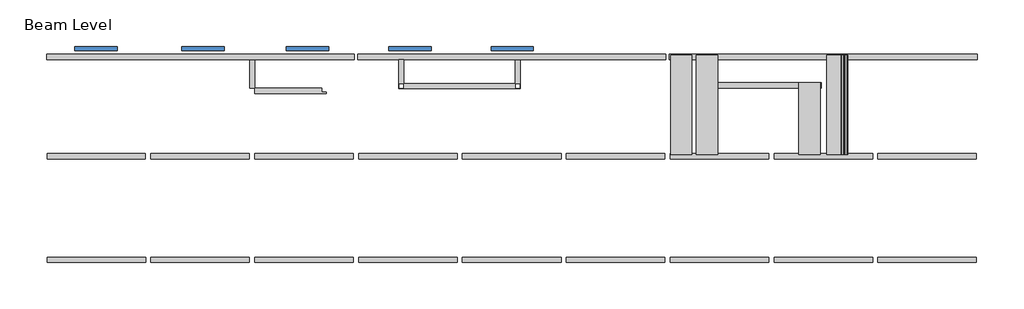
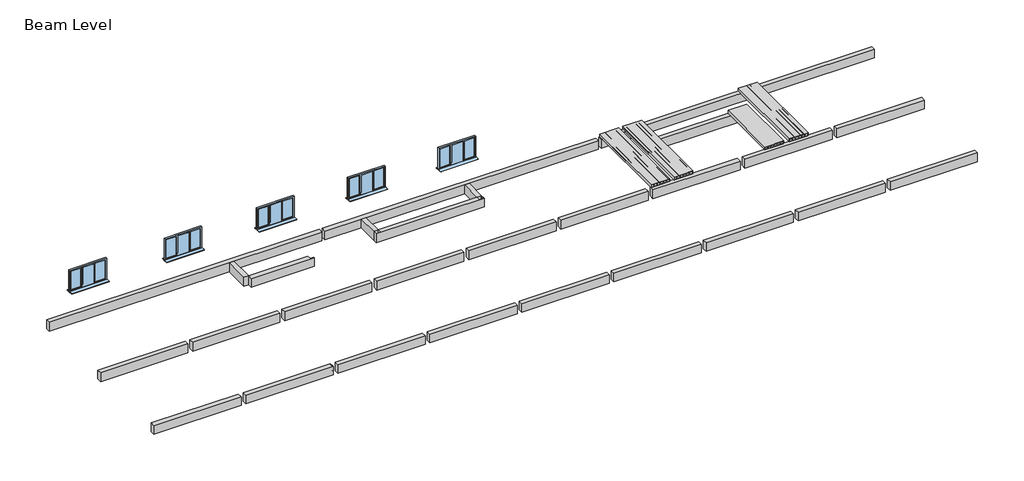
# One storey: 28 beams, 5 windows, 4 proxies.
"""IFC4 building model written with IfcOpenShell, lengths in millimetres."""

import ifcopenshell
import ifcopenshell.guid

model = None  # the IFC model being written
_history = None  # IfcOwnerHistory: only IFC2X3 demands one
_inside = {}  # id of a spatial element -> (the spatial element, [elements in it])
_under = {}  # id of a project, library or spatial element -> (it, [spatial elements below it])
_declared = {}  # id of a project -> (the project, [libraries it declares])
_typed = {}  # id of a type object -> (the type object, [elements of that type])
_made_of = {}  # id of a material, layer set ... -> (it, [elements and type objects made of it])


def new_model(schema):
    """Start an empty IFC model of exactly this schema.

    Asked for "IFC4X3", IfcOpenShell would pick the latest addendum, in which some entities
    have other attributes; the version numbers below select the first issue.
    IFC2X3 requires an IfcOwnerHistory on every rooted entity: one is made here for all.
    """
    global model, _history
    if schema == "IFC4X3":
        model = ifcopenshell.file(schema_version=(4, 3, 0, 0))
    else:
        model = ifcopenshell.file(schema=schema)
    _inside.clear()
    _under.clear()
    _declared.clear()
    _typed.clear()
    _made_of.clear()
    _history = None
    if model.schema == "IFC2X3":
        org = make("IfcOrganization", Name="unknown")
        user = make(
            "IfcPersonAndOrganization",
            ThePerson=make("IfcPerson", FamilyName="unknown"),
            TheOrganization=org,
        )
        app = make(
            "IfcApplication",
            ApplicationDeveloper=org,
            Version="unknown",
            ApplicationFullName="unknown",
            ApplicationIdentifier="unknown",
        )
        _history = make(
            "IfcOwnerHistory",
            OwningUser=user,
            OwningApplication=app,
            ChangeAction="ADDED",
            CreationDate=0,
        )
    return model


def make(cls, **values):
    """One entity of the class cls with the attributes given. An attribute that is None is left unset."""
    return model.create_entity(
        cls, **{name: value for name, value in values.items() if value is not None}
    )


def rooted(cls, **values):
    """An entity with a GlobalId (a new one), such as an element, a storey or a relation."""
    return make(cls, GlobalId=ifcopenshell.guid.new(), OwnerHistory=_history, **values)


def si_unit(unit_type, name, prefix=None):
    """IfcSIUnit, for example si_unit("LENGTHUNIT", "METRE", prefix="MILLI")."""
    return make("IfcSIUnit", UnitType=unit_type, Prefix=prefix, Name=name)


def assignment(units):
    """IfcUnitAssignment: the units of a project."""
    return None if units is None else make("IfcUnitAssignment", Units=units)


def point(xyz):
    """IfcCartesianPoint."""
    return None if xyz is None else make("IfcCartesianPoint", Coordinates=xyz)


def direction(xyz):
    """IfcDirection."""
    return None if xyz is None else make("IfcDirection", DirectionRatios=xyz)


def frame(location, z_axis=None, x_axis=None):
    """IfcAxis2Placement3D, a coordinate frame: its origin and axes. An axis left out is left unset."""
    return make(
        "IfcAxis2Placement3D",
        Location=point(location),
        Axis=direction(z_axis),
        RefDirection=direction(x_axis),
    )


def frame_2d(location, x_axis=None):
    """IfcAxis2Placement2D, a coordinate frame in the plane: its origin and x axis."""
    return make(
        "IfcAxis2Placement2D", Location=point(location), RefDirection=direction(x_axis)
    )


def origin():
    """The frame at (0, 0, 0) with its axes left unset."""
    return frame((0.0, 0.0, 0.0))


def place(relative_to, where):
    """IfcLocalPlacement: puts the frame where relative to a parent placement (None: the world)."""
    return make(
        "IfcLocalPlacement", PlacementRelTo=relative_to, RelativePlacement=where
    )


def context(
    kind, dimensions, precision=None, world=None, true_north=None, identifier=None
):
    """IfcGeometricRepresentationContext, for example the 3D "Model" context."""
    return make(
        "IfcGeometricRepresentationContext",
        ContextIdentifier=identifier,
        ContextType=kind,
        CoordinateSpaceDimension=dimensions,
        Precision=precision,
        WorldCoordinateSystem=world,
        TrueNorth=true_north,
    )


def project(units=None, contexts=None):
    """IfcProject with its units and contexts."""
    return rooted(
        "IfcProject",
        Name="project",
        RepresentationContexts=contexts,
        UnitsInContext=assignment(units),
    )


def spatial(cls, under=None, at=None, **own):
    """A site, building, storey or space (cls), placed at a placement, below another one or the project."""
    s = rooted(cls, ObjectPlacement=at, **own)
    if under is not None:
        _under.setdefault(under.id(), (under, []))[1].append(s)
    return s


def polyline(points):
    """IfcPolyline through the points."""
    return make("IfcPolyline", Points=[point(p) for p in points])


def circle_curve(where, radius):
    """IfcCircle in the frame where."""
    return make("IfcCircle", Position=where, Radius=radius)


def trimmed(basis, trim1, trim2, sense, master):
    """IfcTrimmedCurve: the piece of a basis curve between two trims."""
    return make(
        "IfcTrimmedCurve",
        BasisCurve=basis,
        Trim1=trim1,
        Trim2=trim2,
        SenseAgreement=sense,
        MasterRepresentation=master,
    )


def segment(curve, same_sense, transition):
    """IfcCompositeCurveSegment."""
    return make(
        "IfcCompositeCurveSegment",
        Transition=transition,
        SameSense=same_sense,
        ParentCurve=curve,
    )


def composite_curve(segments, self_intersect=None):
    """IfcCompositeCurve: segments joined end to end."""
    return make("IfcCompositeCurve", Segments=segments, SelfIntersect=self_intersect)


def outline(outer, holes=None, kind="AREA"):
    """IfcArbitraryClosedProfileDef: a profile drawn as a closed curve; with holes, ...WithVoids."""
    if holes is None:
        return make("IfcArbitraryClosedProfileDef", ProfileType=kind, OuterCurve=outer)
    return make(
        "IfcArbitraryProfileDefWithVoids",
        ProfileType=kind,
        OuterCurve=outer,
        InnerCurves=holes,
    )


def extrude(swept, where, along, depth):
    """IfcExtrudedAreaSolid: the profile swept, set in the frame where, extruded along a direction by depth."""
    return make(
        "IfcExtrudedAreaSolid",
        SweptArea=swept,
        Position=where,
        ExtrudedDirection=direction(along),
        Depth=depth,
    )


def faces_of(points, faces, orient=None, outer=None):
    """IfcFace entities. A face is a list of loops; a loop is a list of indices into points, from 0.

    orient and outer hold one flag for each loop. By default every Orientation is true, the
    first loop of a face is its IfcFaceOuterBound and the others are IfcFaceBound.
    """
    made = []
    for i, loops in enumerate(faces):
        bounds = []
        for j, loop in enumerate(loops):
            is_outer = j == 0 if outer is None else outer[i][j]
            bounds.append(
                make(
                    "IfcFaceOuterBound" if is_outer else "IfcFaceBound",
                    Bound=make("IfcPolyLoop", Polygon=[points[k] for k in loop]),
                    Orientation=True if orient is None else orient[i][j],
                )
            )
        made.append(make("IfcFace", Bounds=bounds))
    return made


def faceted_brep(points, faces, orient=None, outer=None, voids=None):
    """IfcFacetedBrep: a solid bounded by flat faces; with voids (closed shells), ...WithVoids."""
    shared = [point(p) for p in points]
    hull = make("IfcClosedShell", CfsFaces=faces_of(shared, faces, orient, outer))
    if voids is None:
        return make("IfcFacetedBrep", Outer=hull)
    return make(
        "IfcFacetedBrepWithVoids",
        Outer=hull,
        Voids=[
            make(cls, CfsFaces=faces_of(shared, fs, o, b)) for cls, fs, o, b in voids
        ],
    )


def shape(context_of_items, identifier, shape_type, items):
    """IfcShapeRepresentation: the items that make up one representation, for example the "Body"."""
    return make(
        "IfcShapeRepresentation",
        ContextOfItems=context_of_items,
        RepresentationIdentifier=identifier,
        RepresentationType=shape_type,
        Items=items,
    )


def source(mapping_origin, context_of_items, identifier, shape_type, items):
    """IfcRepresentationMap: a shape defined once, which mapped items show again and again."""
    return make(
        "IfcRepresentationMap",
        MappingOrigin=mapping_origin,
        MappedRepresentation=shape(context_of_items, identifier, shape_type, items),
    )


def transform(
    local_origin,
    x_axis=None,
    y_axis=None,
    z_axis=None,
    scale=None,
    scale2=None,
    scale3=None,
    uniform=True,
):
    """IfcCartesianTransformationOperator3D, or its non-uniform kind. x_axis, y_axis, z_axis: its Axis1, 2, 3."""
    if uniform:
        return make(
            "IfcCartesianTransformationOperator3D",
            Axis1=direction(x_axis),
            Axis2=direction(y_axis),
            LocalOrigin=point(local_origin),
            Scale=scale,
            Axis3=direction(z_axis),
        )
    return make(
        "IfcCartesianTransformationOperator3DnonUniform",
        Axis1=direction(x_axis),
        Axis2=direction(y_axis),
        LocalOrigin=point(local_origin),
        Scale=scale,
        Axis3=direction(z_axis),
        Scale2=scale2,
        Scale3=scale3,
    )


def mapped(mapping_source, mapping_target):
    """IfcMappedItem: shows the shape of a source again, moved by a transform."""
    return make(
        "IfcMappedItem", MappingSource=mapping_source, MappingTarget=mapping_target
    )


def made_of(thing, what):
    """Note that an element or type object is made of a material, layer set ...; save() writes the relation."""
    if what is not None:
        _made_of.setdefault(what.id(), (what, []))[1].append(thing)
    return thing


def element(
    cls,
    number,
    at=None,
    inside=None,
    cuts=None,
    type_object=None,
    material=None,
    context=None,
    identifier="Body",
    shape_type=None,
    held_by="IfcProductDefinitionShape",
    body=None,
    shapes=None,
    **own,
):
    """One element of the class cls, such as IfcWall. Its Tag is "e" and its number.

    at: its placement. inside: the storey or other place that contains it. cuts: it is an
    opening in that element (IfcRelVoidsElement). A single representation is given by context,
    identifier, shape_type and body (its items); several are given by shapes. held_by: the class
    of the entity that holds the representations. save() writes the other relations.
    """
    e = rooted(cls, Tag="e%d" % number, ObjectPlacement=at, **own)
    if body is not None:
        shapes = [shape(context, identifier, shape_type, body)]
    if shapes is not None:
        e.Representation = make(held_by, Representations=shapes)
    if inside is not None:
        _inside.setdefault(inside.id(), (inside, []))[1].append(e)
    if cuts is not None:
        rooted(
            "IfcRelVoidsElement", RelatingBuildingElement=cuts, RelatedOpeningElement=e
        )
    if type_object is not None:
        _typed.setdefault(type_object.id(), (type_object, []))[1].append(e)
    return made_of(e, material)


def aggregate(whole, parts):
    """IfcRelAggregates: a whole, such as a stair, and the parts it consists of."""
    return rooted("IfcRelAggregates", RelatingObject=whole, RelatedObjects=parts)


def save(model, path):
    """Write the relations noted so far, then the file.

    IfcRelAggregates (storeys below a building ...), IfcRelContainedInSpatialStructure (elements
    in a storey), IfcRelDefinesByType, IfcRelAssociatesMaterial and IfcRelDeclares: one each for
    every whole, place, type object, material and project.
    """
    for whole, parts in _under.values():
        aggregate(whole, parts)
    for where, things in _inside.values():
        rooted(
            "IfcRelContainedInSpatialStructure",
            RelatedElements=things,
            RelatingStructure=where,
        )
    for kind, things in _typed.values():
        rooted("IfcRelDefinesByType", RelatedObjects=things, RelatingType=kind)
    for what, things in _made_of.values():
        rooted("IfcRelAssociatesMaterial", RelatedObjects=things, RelatingMaterial=what)
    for by, libraries in _declared.values():
        rooted("IfcRelDeclares", RelatingContext=by, RelatedDefinitions=libraries)
    model.write(path)


def asb_beams_300asb153_cd404b0f(model_context):
    return source(origin(), model_context, "Body", "SweptSolid", [
        extrude(outline(composite_curve([segment(polyline([(95.0, 174.0), (95.0, 150.0), (40.5, 150.0)]), True, "CONTINUOUS"), segment(trimmed(circle_curve(frame_2d((40.5, 123.0)), 27.0), [point((40.5, 150.0))], [point((13.5, 123.0))], True, "CARTESIAN"), True, "CONTINUOUS"), segment(polyline([(13.5, 123.0), (13.5, -85.0)]), True, "CONTINUOUS"), segment(trimmed(circle_curve(frame_2d((40.5, -85.0)), 27.0), [point((13.5, -85.0))], [point((40.5, -112.0))], True, "CARTESIAN"), True, "CONTINUOUS"), segment(polyline([(40.5, -112.0), (150.0, -112.0), (150.0, -136.0), (-150.0, -136.0), (-150.0, -112.0), (-40.5, -112.0)]), True, "CONTINUOUS"), segment(trimmed(circle_curve(frame_2d((-40.5, -85.0)), 27.0), [point((-40.5, -112.0))], [point((-13.5, -85.0))], True, "CARTESIAN"), True, "CONTINUOUS"), segment(polyline([(-13.5, -85.0), (-13.5, 123.0)]), True, "CONTINUOUS"), segment(trimmed(circle_curve(frame_2d((-40.5, 123.0)), 27.0), [point((-13.5, 123.0))], [point((-40.5, 150.0))], True, "CARTESIAN"), True, "CONTINUOUS"), segment(polyline([(-40.5, 150.0), (-95.0, 150.0), (-95.0, 174.0), (95.0, 174.0)]), True, "CONTINUOUS")], self_intersect=False)), frame((-176.5, 0.0, 0.0), z_axis=(1.0, 0.0, 0.0), x_axis=(0.0, 1.0, 0.0)), (0.0, 0.0, 1.0), 36.0),
    ])


def hollow_core_b1c9e8cf(model_context):
    return source(origin(), model_context, "Body", "SweptSolid", [
        extrude(outline(polyline([(-609.6, 100.0), (609.6, 100.0), (609.6, -100.0), (-609.6, -100.0), (-609.6, 100.0)]), holes=[composite_curve([segment(trimmed(circle_curve(frame_2d((508.0, 0.0)), 60.0), [point((448.0, 0.0))], [point((568.0, 0.0))], True, "CARTESIAN"), True, "CONTINUOUS"), segment(trimmed(circle_curve(frame_2d((508.0, 0.0)), 60.0), [point((568.0, 0.0))], [point((448.0, 0.0))], True, "CARTESIAN"), True, "CONTINUOUS")], self_intersect=False), composite_curve([segment(trimmed(circle_curve(frame_2d((-508.0, 0.0)), 60.0), [point((-568.0, 0.0))], [point((-448.0, 0.0))], True, "CARTESIAN"), True, "CONTINUOUS"), segment(trimmed(circle_curve(frame_2d((-508.0, 0.0)), 60.0), [point((-448.0, 0.0))], [point((-568.0, 0.0))], True, "CARTESIAN"), True, "CONTINUOUS")], self_intersect=False), composite_curve([segment(trimmed(circle_curve(frame_2d((304.8, 0.0)), 60.0), [point((244.8, 0.0))], [point((364.8, 0.0))], True, "CARTESIAN"), True, "CONTINUOUS"), segment(trimmed(circle_curve(frame_2d((304.8, 0.0)), 60.0), [point((364.8, 0.0))], [point((244.8, 0.0))], True, "CARTESIAN"), True, "CONTINUOUS")], self_intersect=False), composite_curve([segment(trimmed(circle_curve(frame_2d((101.6, 0.0)), 60.0), [point((41.6, 0.0))], [point((161.6, 0.0))], True, "CARTESIAN"), True, "CONTINUOUS"), segment(trimmed(circle_curve(frame_2d((101.6, 0.0)), 60.0), [point((161.6, 0.0))], [point((41.6, 0.0))], True, "CARTESIAN"), True, "CONTINUOUS")], self_intersect=False), composite_curve([segment(trimmed(circle_curve(frame_2d((-101.6, 0.0)), 60.0), [point((-161.6, 0.0))], [point((-41.6, 0.0))], True, "CARTESIAN"), True, "CONTINUOUS"), segment(trimmed(circle_curve(frame_2d((-101.6, 0.0)), 60.0), [point((-41.6, 0.0))], [point((-161.6, 0.0))], True, "CARTESIAN"), True, "CONTINUOUS")], self_intersect=False), composite_curve([segment(trimmed(circle_curve(frame_2d((-304.8, 0.0)), 60.0), [point((-364.8, 0.0))], [point((-244.8, 0.0))], True, "CARTESIAN"), True, "CONTINUOUS"), segment(trimmed(circle_curve(frame_2d((-304.8, 0.0)), 60.0), [point((-244.8, 0.0))], [point((-364.8, 0.0))], True, "CARTESIAN"), True, "CONTINUOUS")], self_intersect=False)]), frame((0.0, 0.0, 0.0), z_axis=(1.0, 0.0, 0.0), x_axis=(0.0, 1.0, 0.0)), (0.0, 0.0, 1.0), 5760.0),
    ])


def hollow_core_a6975cb3(model_context):
    return source(origin(), model_context, "Body", "SweptSolid", [
        extrude(outline(polyline([(-609.6, 100.0), (609.6, 100.0), (609.6, -100.0), (-609.6, -100.0), (-609.6, 100.0)]), holes=[composite_curve([segment(trimmed(circle_curve(frame_2d((508.0, 0.0)), 60.0), [point((448.0, 0.0))], [point((568.0, 0.0))], True, "CARTESIAN"), True, "CONTINUOUS"), segment(trimmed(circle_curve(frame_2d((508.0, 0.0)), 60.0), [point((568.0, 0.0))], [point((448.0, 0.0))], True, "CARTESIAN"), True, "CONTINUOUS")], self_intersect=False), composite_curve([segment(trimmed(circle_curve(frame_2d((-508.0, 0.0)), 60.0), [point((-568.0, 0.0))], [point((-448.0, 0.0))], True, "CARTESIAN"), True, "CONTINUOUS"), segment(trimmed(circle_curve(frame_2d((-508.0, 0.0)), 60.0), [point((-448.0, 0.0))], [point((-568.0, 0.0))], True, "CARTESIAN"), True, "CONTINUOUS")], self_intersect=False), composite_curve([segment(trimmed(circle_curve(frame_2d((304.8, 0.0)), 60.0), [point((244.8, 0.0))], [point((364.8, 0.0))], True, "CARTESIAN"), True, "CONTINUOUS"), segment(trimmed(circle_curve(frame_2d((304.8, 0.0)), 60.0), [point((364.8, 0.0))], [point((244.8, 0.0))], True, "CARTESIAN"), True, "CONTINUOUS")], self_intersect=False), composite_curve([segment(trimmed(circle_curve(frame_2d((101.6, 0.0)), 60.0), [point((41.6, 0.0))], [point((161.6, 0.0))], True, "CARTESIAN"), True, "CONTINUOUS"), segment(trimmed(circle_curve(frame_2d((101.6, 0.0)), 60.0), [point((161.6, 0.0))], [point((41.6, 0.0))], True, "CARTESIAN"), True, "CONTINUOUS")], self_intersect=False), composite_curve([segment(trimmed(circle_curve(frame_2d((-101.6, 0.0)), 60.0), [point((-161.6, 0.0))], [point((-41.6, 0.0))], True, "CARTESIAN"), True, "CONTINUOUS"), segment(trimmed(circle_curve(frame_2d((-101.6, 0.0)), 60.0), [point((-41.6, 0.0))], [point((-161.6, 0.0))], True, "CARTESIAN"), True, "CONTINUOUS")], self_intersect=False), composite_curve([segment(trimmed(circle_curve(frame_2d((-304.8, 0.0)), 60.0), [point((-364.8, 0.0))], [point((-244.8, 0.0))], True, "CARTESIAN"), True, "CONTINUOUS"), segment(trimmed(circle_curve(frame_2d((-304.8, 0.0)), 60.0), [point((-244.8, 0.0))], [point((-364.8, 0.0))], True, "CARTESIAN"), True, "CONTINUOUS")], self_intersect=False)]), frame((0.0, 0.0, 0.0), z_axis=(1.0, 0.0, 0.0), x_axis=(0.0, 1.0, 0.0)), (0.0, 0.0, 1.0), 4157.5),
    ])


def windows_commercial_ff_rear_windows_2400long_x_1500high_d88e899e(model_context):
    return source(origin(), model_context, "Body", "SolidModel", [
        extrude(outline(polyline([(-1860.0, -231.5434322), (-1860.0, -138.5434322), (-1860.0, 8.4565678), (590.0, 8.4565678), (590.0, -138.5434322), (590.0, -231.5434322), (-1860.0, -231.5434322)])), frame((0.0, 0.0, 636.5715519), z_axis=(0.0, 0.0, 1.0), x_axis=(1.0, 0.0, 0.0)), (0.0, 0.0, 1.0), 26.4284481),
        extrude(outline(polyline([(495.0, 87.4565678), (-190.0, 87.4565678), (-190.0, 111.4565678), (495.0, 111.4565678), (495.0, 87.4565678)])), frame((0.0, 0.0, 693.0), z_axis=(0.0, 0.0, 1.0), x_axis=(1.0, 0.0, 0.0)), (0.0, 0.0, 1.0), 1337.0),
        extrude(outline(polyline([(-1020.0, 47.4565678), (-250.0, 47.4565678), (-250.0, 23.4565678), (-1020.0, 23.4565678), (-1020.0, 47.4565678)])), frame((0.0, 0.0, 663.0), z_axis=(0.0, 0.0, 1.0), x_axis=(1.0, 0.0, 0.0)), (0.0, 0.0, 1.0), 1397.0),
        extrude(outline(polyline([(-1080.0, 87.4565678), (-1765.0, 87.4565678), (-1765.0, 111.4565678), (-1080.0, 111.4565678), (-1080.0, 87.4565678)])), frame((0.0, 0.0, 693.0), z_axis=(0.0, 0.0, 1.0), x_axis=(1.0, 0.0, 0.0)), (0.0, 0.0, 1.0), 1337.0),
        faceted_brep([(-1835.0, 5.4565678, 663.0), (-1775.0, 5.4565678, 663.0), (-1775.0, 5.4565678, 2040.0), (-1068.0, 5.4565678, 2040.0), (-1068.0, 5.4565678, 863.0), (-1010.0, 5.4565678, 863.0), (-1010.0, 5.4565678, 2040.0), (-260.0, 5.4565678, 2040.0), (-260.0, 5.4565678, 663.0), (-202.0, 5.4565678, 663.0), (-202.0, 5.4565678, 2040.0), (505.0, 5.4565678, 2040.0), (505.0, 5.4565678, 663.0), (565.0, 5.4565678, 663.0), (565.0, 5.4565678, 2100.0), (-1835.0, 5.4565678, 2100.0), (-1835.0, 123.4565678, 2100.0), (-1835.0, 123.4565678, 663.0), (-1835.0, 73.4565678, 663.0), (-1835.0, 8.4565678, 663.0), (-1795.0, 123.4565678, 663.0), (565.0, 123.4565678, 2100.0), (565.0, 123.4565678, 663.0), (525.0, 123.4565678, 663.0), (525.0, 123.4565678, 2060.0), (-220.0, 123.4565678, 2060.0), (-220.0, 123.4565678, 663.0), (-260.0, 123.4565678, 663.0), (-260.0, 123.4565678, 2060.0), (-1010.0, 123.4565678, 2060.0), (-1010.0, 123.4565678, 863.0), (-1050.0, 123.4565678, 863.0), (-1050.0, 123.4565678, 2060.0), (-1795.0, 123.4565678, 2060.0), (-1795.0, 23.4565678, 2060.0), (-1795.0, 23.4565678, 663.0), (-1795.0, 73.4565678, 663.0), (-1050.0, 23.4565678, 2060.0), (-1050.0, 23.4565678, 863.0), (-1068.0, 23.4565678, 863.0), (-1068.0, 23.4565678, 2040.0), (-1775.0, 23.4565678, 2040.0), (-1775.0, 23.4565678, 663.0), (525.0, 23.4565678, 2060.0), (525.0, 23.4565678, 663.0), (505.0, 23.4565678, 663.0), (505.0, 23.4565678, 2040.0), (-202.0, 23.4565678, 2040.0), (-202.0, 23.4565678, 663.0), (-220.0, 23.4565678, 663.0), (-220.0, 23.4565678, 2060.0), (-1010.0, 23.4565678, 863.0), (-1020.0, 23.4565678, 863.0), (-1020.0, 23.4565678, 2060.0), (-250.0, 23.4565678, 2060.0), (-250.0, 23.4565678, 663.0), (-260.0, 23.4565678, 663.0), (-260.0, 23.4565678, 2040.0), (-1010.0, 23.4565678, 2040.0), (-1775.0, 8.4565678, 663.0), (-1010.0, 47.4565678, 2060.0), (-260.0, 47.4565678, 2060.0), (-250.0, 47.4565678, 2060.0), (-1020.0, 47.4565678, 2060.0), (565.0, 8.4565678, 663.0), (565.0, 73.4565678, 663.0), (525.0, 73.4565678, 663.0), (505.0, 8.4565678, 663.0), (-1010.0, 47.4565678, 863.0), (-1020.0, 47.4565678, 863.0), (-250.0, 47.4565678, 663.0), (-260.0, 47.4565678, 663.0), (-260.0, 73.4565678, 663.0), (-220.0, 73.4565678, 663.0), (-202.0, 8.4565678, 663.0), (-260.0, 8.4565678, 663.0), (590.0, 248.4565678, 600.0), (590.0, 8.4565678, 600.0), (-1860.0, 8.4565678, 600.0), (-1860.0, 248.4565678, 600.0), (590.0, 248.4565678, 637.0666405), (-1860.0, 248.4565678, 637.0666405), (590.0, 73.4565678, 649.0962075), (-1860.0, 73.4565678, 649.0962075), (590.0, 8.4565678, 663.0), (590.0, 73.4565678, 663.0), (-1860.0, 73.4565678, 663.0), (-1860.0, 8.4565678, 663.0)], [[[0, 1, 2, 3, 4, 5, 6, 7, 8, 9, 10, 11, 12, 13, 14, 15]], [[0, 15, 16, 17, 18, 19]], [[20, 17, 16, 21, 22, 23, 24, 25, 26, 27, 28, 29, 30, 31, 32, 33]], [[20, 33, 34, 35, 36]], [[35, 34, 37, 38, 39, 40, 41, 42]], [[43, 44, 45, 46, 47, 48, 49, 50]], [[51, 52, 53, 54, 55, 56, 57, 58]], [[2, 1, 59, 42, 41]], [[15, 14, 21, 16]], [[34, 33, 32, 37]], [[24, 43, 50, 25]], [[60, 29, 28, 61, 62, 54, 53, 63]], [[2, 41, 40, 3]], [[46, 11, 10, 47]], [[6, 58, 57, 7]], [[14, 13, 64, 65, 22, 21]], [[24, 23, 66, 44, 43]], [[12, 11, 46, 45, 67]], [[5, 51, 58, 6]], [[39, 4, 3, 40]], [[31, 38, 37, 32]], [[68, 30, 29, 60]], [[69, 68, 60, 63]], [[52, 69, 63, 53]], [[62, 70, 55, 54]], [[70, 62, 61, 71]], [[71, 61, 28, 27, 72]], [[26, 25, 50, 49, 73]], [[10, 9, 74, 48, 47]], [[8, 7, 57, 56, 75]], [[76, 77, 78, 79]], [[80, 76, 79, 81]], [[82, 80, 81, 83]], [[84, 85, 65, 64]], [[86, 87, 19, 18]], [[72, 36, 35, 42, 59, 75, 56, 55, 70, 71]], [[66, 73, 49, 48, 74, 67, 45, 44]], [[17, 20, 36, 18]], [[1, 0, 19, 59]], [[23, 22, 65, 66]], [[13, 12, 67, 64]], [[51, 5, 4, 39, 38, 31, 30, 68, 69, 52]], [[27, 26, 73, 72]], [[9, 8, 75, 74]], [[84, 77, 76, 80, 82, 85]], [[87, 86, 83, 81, 79, 78]], [[85, 82, 83, 86, 18, 36, 72, 73, 66, 65]], [[77, 84, 64, 67, 74, 75, 59, 19, 87, 78]]]),
        faceted_brep([(-1050.0, 23.4565678, 2060.0), (-1050.0, 93.4565678, 2060.0), (-1795.0, 93.4565678, 2060.0), (-1795.0, 23.4565678, 2060.0), (-1090.0, 37.9494677, 2020.0), (-1079.8519623, 23.4565678, 2030.1480377), (-1765.1480377, 23.4565678, 2030.1480377), (-1755.0, 37.9494677, 2020.0), (-1090.0, 87.4565678, 2020.0), (-1755.0, 87.4565678, 2020.0), (-1080.0, 111.4565678, 2030.0), (-1080.0, 87.4565678, 2030.0), (-1765.0, 87.4565678, 2030.0), (-1765.0, 111.4565678, 2030.0), (-1090.0, 129.2300705, 2020.0), (-1090.0, 111.4565678, 2020.0), (-1755.0, 111.4565678, 2020.0), (-1755.0, 129.2300705, 2020.0), (-1071.1854344, 135.0035732, 2038.8145656), (-1773.8145656, 135.0035732, 2038.8145656), (-1795.0, 93.4565678, 663.0), (-1795.0, 23.4565678, 663.0), (-1765.1480377, 23.4565678, 692.8519623), (-1755.0, 37.9494677, 703.0), (-1755.0, 87.4565678, 703.0), (-1765.0, 87.4565678, 693.0), (-1765.0, 111.4565678, 693.0), (-1755.0, 111.4565678, 703.0), (-1755.0, 129.2300705, 703.0), (-1773.8145656, 135.0035732, 684.1854344), (-1050.0, 93.4565678, 663.0), (-1050.0, 23.4565678, 663.0), (-1079.8519623, 23.4565678, 692.8519623), (-1090.0, 37.9494677, 703.0), (-1090.0, 87.4565678, 703.0), (-1080.0, 87.4565678, 693.0), (-1080.0, 111.4565678, 693.0), (-1090.0, 111.4565678, 703.0), (-1090.0, 129.2300705, 703.0), (-1071.1854344, 135.0035732, 684.1854344), (-1040.0, 135.0035732, 653.0), (-1805.0, 135.0035732, 653.0), (-1805.0, 135.0035732, 2070.0), (-1040.0, 135.0035732, 2070.0), (-1040.0, 93.4565678, 2070.0), (-1805.0, 93.4565678, 2070.0), (-1805.0, 93.4565678, 653.0), (-1040.0, 93.4565678, 653.0)], [[[0, 1, 2, 3]], [[4, 5, 6, 7]], [[8, 4, 7, 9]], [[10, 11, 12, 13]], [[14, 15, 16, 17]], [[18, 14, 17, 19]], [[3, 2, 20, 21]], [[7, 6, 22, 23]], [[9, 7, 23, 24]], [[13, 12, 25, 26]], [[17, 16, 27, 28]], [[19, 17, 28, 29]], [[21, 20, 30, 31]], [[0, 3, 21, 31], [32, 22, 6, 5]], [[23, 22, 32, 33]], [[24, 23, 33, 34]], [[35, 25, 12, 11], [8, 9, 24, 34]], [[26, 25, 35, 36]], [[10, 13, 26, 36], [37, 27, 16, 15]], [[28, 27, 37, 38]], [[29, 28, 38, 39]], [[40, 41, 42, 43], [18, 19, 29, 39]], [[30, 1, 0, 31]], [[33, 32, 5, 4]], [[34, 33, 4, 8]], [[36, 35, 11, 10]], [[38, 37, 15, 14]], [[39, 38, 14, 18]], [[44, 43, 42, 45]], [[45, 42, 41, 46]], [[46, 41, 40, 47]], [[47, 40, 43, 44]], [[45, 46, 47, 44], [1, 30, 20, 2]]]),
        faceted_brep([(-230.0, 87.4565678, 2070.0), (-230.0, 129.2300705, 2070.0), (-230.0, 129.2300705, 653.0), (-230.0, 87.4565678, 653.0), (-220.0, 23.4565678, 2060.0), (-220.0, 87.4565678, 2060.0), (-220.0, 87.4565678, 663.0), (-220.0, 23.4565678, 663.0), (-180.0, 37.9494677, 2020.0), (-190.1480377, 23.4565678, 2030.1480377), (-190.1480377, 23.4565678, 692.8519623), (-180.0, 37.9494677, 703.0), (-180.0, 87.4565678, 2020.0), (-180.0, 87.4565678, 703.0), (-190.0, 111.4565678, 2030.0), (-190.0, 87.4565678, 2030.0), (-190.0, 87.4565678, 693.0), (-190.0, 111.4565678, 693.0), (-180.0, 129.2300705, 2020.0), (-180.0, 111.4565678, 2020.0), (-180.0, 111.4565678, 703.0), (-180.0, 129.2300705, 703.0), (-197.4457548, 135.0035732, 2037.4457548), (-197.4457548, 135.0035732, 685.5542452), (-219.2153903, 135.0035732, 2059.2153903), (-219.2153903, 135.0035732, 663.7846097), (535.0, 129.2300705, 653.0), (535.0, 87.4565678, 653.0), (525.0, 87.4565678, 663.0), (525.0, 23.4565678, 663.0), (495.1480377, 23.4565678, 692.8519623), (485.0, 37.9494677, 703.0), (485.0, 87.4565678, 703.0), (495.0, 87.4565678, 693.0), (495.0, 111.4565678, 693.0), (485.0, 111.4565678, 703.0), (485.0, 129.2300705, 703.0), (502.4457548, 135.0035732, 685.5542452), (524.2153903, 135.0035732, 663.7846097), (535.0, 129.2300705, 2070.0), (535.0, 87.4565678, 2070.0), (525.0, 87.4565678, 2060.0), (525.0, 23.4565678, 2060.0), (495.1480377, 23.4565678, 2030.1480377), (485.0, 37.9494677, 2020.0), (485.0, 87.4565678, 2020.0), (495.0, 87.4565678, 2030.0), (495.0, 111.4565678, 2030.0), (485.0, 111.4565678, 2020.0), (485.0, 129.2300705, 2020.0), (502.4457548, 135.0035732, 2037.4457548), (524.2153903, 135.0035732, 2059.2153903)], [[[0, 1, 2, 3]], [[4, 5, 6, 7]], [[8, 9, 10, 11]], [[12, 8, 11, 13]], [[14, 15, 16, 17]], [[18, 19, 20, 21]], [[22, 18, 21, 23]], [[1, 24, 25, 2]], [[3, 2, 26, 27]], [[7, 6, 28, 29]], [[11, 10, 30, 31]], [[13, 11, 31, 32]], [[17, 16, 33, 34]], [[21, 20, 35, 36]], [[23, 21, 36, 37]], [[2, 25, 38, 26]], [[27, 26, 39, 40]], [[29, 28, 41, 42]], [[31, 30, 43, 44]], [[32, 31, 44, 45]], [[34, 33, 46, 47]], [[36, 35, 48, 49]], [[37, 36, 49, 50]], [[26, 38, 51, 39]], [[40, 39, 1, 0]], [[42, 41, 5, 4]], [[7, 29, 42, 4], [9, 43, 30, 10]], [[44, 43, 9, 8]], [[45, 44, 8, 12]], [[15, 46, 33, 16], [13, 32, 45, 12]], [[47, 46, 15, 14]], [[17, 34, 47, 14], [19, 48, 35, 20]], [[49, 48, 19, 18]], [[50, 49, 18, 22]], [[24, 51, 38, 25], [23, 37, 50, 22]], [[39, 51, 24, 1]], [[3, 27, 40, 0], [5, 41, 28, 6]]]),
    ])


model = new_model("IFC4")

# Units and contexts
model_context = context("Model", 3, world=origin())
ifc_project = project(units=[si_unit("LENGTHUNIT", "METRE", prefix="MILLI")], contexts=[model_context])

# Site, building, storey
site = spatial("IfcSite", under=ifc_project)
building = spatial("IfcBuilding", under=site)
storey = spatial("IfcBuildingStorey", under=building, Name="Beam Level", Elevation=3700.0)

# Beams
placement = place(None, origin())
asb_beams_300asb153_shape = asb_beams_300asb153_cd404b0f(model_context)
element("IfcBeam", 1, ObjectType="ASB-Beams : 300ASB153", at=placement, inside=storey, context=model_context, shape_type="MappedRepresentation", body=[
    mapped(asb_beams_300asb153_shape, transform((4837.4196543, -5058.7619082, 3526.0), x_axis=(1.0, 0.0, 0.0), y_axis=(0.0, 1.0, 0.0), z_axis=(0.0, 0.0, 1.0))),
])
element("IfcBeam", 2, ObjectType="Concrete - Rectangular Beam : 300 x 600mm", at=placement, inside=storey, context=model_context, shape_type="SweptSolid", body=[
    extrude(outline(polyline([(-1300.8053457, 1091.2380918), (-1300.8053457, 791.2380918), (-6984.8053457, 791.2380918), (-6984.8053457, 1091.2380918), (-1300.8053457, 1091.2380918)])), frame((0.0, 0.0, 3100.0), z_axis=(0.0, 0.0, 1.0), x_axis=(1.0, 0.0, 0.0)), (0.0, 0.0, 1.0), 600.0),
])
element("IfcBeam", 3, ObjectType="Concrete - Rectangular Beam : 300 x 600mm", at=placement, inside=storey, context=model_context, shape_type="SweptSolid", body=[
    extrude(outline(polyline([(-985.6053457, 791.2380918), (-985.6053457, 1091.2380918), (4710.4446543, 1091.2380918), (4710.4446543, 791.2380918), (-985.6053457, 791.2380918)])), frame((0.0, 0.0, 3100.0), z_axis=(0.0, 0.0, 1.0), x_axis=(1.0, 0.0, 0.0)), (0.0, 0.0, 1.0), 600.0),
])
element("IfcBeam", 4, ObjectType="Concrete - Rectangular Beam : 300 x 600mm", at=placement, inside=storey, context=model_context, shape_type="SweptSolid", body=[
    extrude(outline(polyline([(10705.4946543, 1091.2380918), (10705.4946543, 791.2380918), (5010.4446543, 791.2380918), (5010.4446543, 1091.2380918), (10705.4946543, 1091.2380918)])), frame((0.0, 0.0, 3100.0), z_axis=(0.0, 0.0, 1.0), x_axis=(1.0, 0.0, 0.0)), (0.0, 0.0, 1.0), 600.0),
])
element("IfcBeam", 5, ObjectType="Concrete - Rectangular Beam : 300 x 600mm", at=placement, inside=storey, context=model_context, shape_type="SweptSolid", body=[
    extrude(outline(polyline([(-6984.6053457, -5208.7619082), (-6984.6053457, -4908.7619082), (-1289.5553457, -4908.7619082), (-1289.5553457, -5208.7619082), (-6984.6053457, -5208.7619082)])), frame((0.0, 0.0, 3100.0), z_axis=(0.0, 0.0, 1.0), x_axis=(1.0, 0.0, 0.0)), (0.0, 0.0, 1.0), 600.0),
])
element("IfcBeam", 6, ObjectType="Concrete - Rectangular Beam : 300 x 600mm", at=placement, inside=storey, context=model_context, shape_type="SweptSolid", body=[
    extrude(outline(polyline([(-985.6053457, -5208.7619082), (-985.6053457, -4908.7619082), (4710.4446543, -4908.7619082), (4710.4446543, -5208.7619082), (-985.6053457, -5208.7619082)])), frame((0.0, 0.0, 3100.0), z_axis=(0.0, 0.0, 1.0), x_axis=(1.0, 0.0, 0.0)), (0.0, 0.0, 1.0), 600.0),
])
element("IfcBeam", 7, ObjectType="Concrete - Rectangular Beam : 300 x 600mm", at=placement, inside=storey, context=model_context, shape_type="SweptSolid", body=[
    extrude(outline(polyline([(10705.4946543, -4908.7619082), (10705.4946543, -5208.7619082), (5010.4446543, -5208.7619082), (5010.4446543, -4908.7619082), (10705.4946543, -4908.7619082)])), frame((0.0, 0.0, 3100.0), z_axis=(0.0, 0.0, 1.0), x_axis=(1.0, 0.0, 0.0)), (0.0, 0.0, 1.0), 600.0),
])
element("IfcBeam", 8, ObjectType="Concrete - Rectangular Beam : 300 x 600mm", at=placement, inside=storey, context=model_context, shape_type="SweptSolid", body=[
    extrude(outline(polyline([(16699.1946543, 1091.2380918), (16699.1946543, 791.2380918), (11015.1946543, 791.2380918), (11015.1946543, 1091.2380918), (16699.1946543, 1091.2380918)])), frame((0.0, 0.0, 3100.0), z_axis=(0.0, 0.0, 1.0), x_axis=(1.0, 0.0, 0.0)), (0.0, 0.0, 1.0), 600.0),
])
element("IfcBeam", 9, ObjectType="Concrete - Rectangular Beam : 300 x 600mm", at=placement, inside=storey, context=model_context, shape_type="SweptSolid", body=[
    extrude(outline(polyline([(17014.3946543, 791.2380918), (17014.3946543, 1091.2380918), (22710.4446543, 1091.2380918), (22710.4446543, 791.2380918), (17014.3946543, 791.2380918)])), frame((0.0, 0.0, 3100.0), z_axis=(0.0, 0.0, 1.0), x_axis=(1.0, 0.0, 0.0)), (0.0, 0.0, 1.0), 600.0),
])
element("IfcBeam", 10, ObjectType="Concrete - Rectangular Beam : 300 x 600mm", at=placement, inside=storey, context=model_context, shape_type="SweptSolid", body=[
    extrude(outline(polyline([(28705.4946543, 1091.2380918), (28705.4946543, 791.2380918), (23010.4446543, 791.2380918), (23010.4446543, 1091.2380918), (28705.4946543, 1091.2380918)])), frame((0.0, 0.0, 3100.0), z_axis=(0.0, 0.0, 1.0), x_axis=(1.0, 0.0, 0.0)), (0.0, 0.0, 1.0), 600.0),
])
element("IfcBeam", 11, ObjectType="Concrete - Rectangular Beam : 300 x 600mm", at=placement, inside=storey, context=model_context, shape_type="SweptSolid", body=[
    extrude(outline(polyline([(11015.3946543, -5208.7619082), (11015.3946543, -4908.7619082), (16710.4446543, -4908.7619082), (16710.4446543, -5208.7619082), (11015.3946543, -5208.7619082)])), frame((0.0, 0.0, 3100.0), z_axis=(0.0, 0.0, 1.0), x_axis=(1.0, 0.0, 0.0)), (0.0, 0.0, 1.0), 600.0),
])
element("IfcBeam", 12, ObjectType="Concrete - Rectangular Beam : 300 x 600mm", at=placement, inside=storey, context=model_context, shape_type="SweptSolid", body=[
    extrude(outline(polyline([(17014.3946543, -5208.7619082), (17014.3946543, -4908.7619082), (22710.4446543, -4908.7619082), (22710.4446543, -5208.7619082), (17014.3946543, -5208.7619082)])), frame((0.0, 0.0, 3100.0), z_axis=(0.0, 0.0, 1.0), x_axis=(1.0, 0.0, 0.0)), (0.0, 0.0, 1.0), 600.0),
])
element("IfcBeam", 13, ObjectType="Concrete - Rectangular Beam : 300 x 600mm", at=placement, inside=storey, context=model_context, shape_type="SweptSolid", body=[
    extrude(outline(polyline([(28705.4946543, -4908.7619082), (28705.4946543, -5208.7619082), (23010.4446543, -5208.7619082), (23010.4446543, -4908.7619082), (28705.4946543, -4908.7619082)])), frame((0.0, 0.0, 3100.0), z_axis=(0.0, 0.0, 1.0), x_axis=(1.0, 0.0, 0.0)), (0.0, 0.0, 1.0), 600.0),
])
element("IfcBeam", 14, ObjectType="Concrete - Rectangular Beam : 300 x 600mm", at=placement, inside=storey, context=model_context, shape_type="SweptSolid", body=[
    extrude(outline(polyline([(34699.1946543, 1091.2380918), (34699.1946543, 791.2380918), (29015.1946543, 791.2380918), (29015.1946543, 1091.2380918), (34699.1946543, 1091.2380918)])), frame((0.0, 0.0, 3100.0), z_axis=(0.0, 0.0, 1.0), x_axis=(1.0, 0.0, 0.0)), (0.0, 0.0, 1.0), 600.0),
])
element("IfcBeam", 15, ObjectType="Concrete - Rectangular Beam : 300 x 600mm", at=placement, inside=storey, context=model_context, shape_type="SweptSolid", body=[
    extrude(outline(polyline([(35014.3946543, 791.2380918), (35014.3946543, 1091.2380918), (40710.4446543, 1091.2380918), (40710.4446543, 791.2380918), (35014.3946543, 791.2380918)])), frame((0.0, 0.0, 3100.0), z_axis=(0.0, 0.0, 1.0), x_axis=(1.0, 0.0, 0.0)), (0.0, 0.0, 1.0), 600.0),
])
element("IfcBeam", 16, ObjectType="Concrete - Rectangular Beam : 300 x 600mm", at=placement, inside=storey, context=model_context, shape_type="SweptSolid", body=[
    extrude(outline(polyline([(46705.4946543, 1091.2380918), (46705.4946543, 791.2380918), (41010.4446543, 791.2380918), (41010.4446543, 1091.2380918), (46705.4946543, 1091.2380918)])), frame((0.0, 0.0, 3100.0), z_axis=(0.0, 0.0, 1.0), x_axis=(1.0, 0.0, 0.0)), (0.0, 0.0, 1.0), 600.0),
])
element("IfcBeam", 17, ObjectType="Concrete - Rectangular Beam : 300 x 600mm", at=placement, inside=storey, context=model_context, shape_type="SweptSolid", body=[
    extrude(outline(polyline([(29015.3946543, -5208.7619082), (29015.3946543, -4908.7619082), (34710.4446543, -4908.7619082), (34710.4446543, -5208.7619082), (29015.3946543, -5208.7619082)])), frame((0.0, 0.0, 3100.0), z_axis=(0.0, 0.0, 1.0), x_axis=(1.0, 0.0, 0.0)), (0.0, 0.0, 1.0), 600.0),
])
element("IfcBeam", 18, ObjectType="Concrete - Rectangular Beam : 300 x 600mm", at=placement, inside=storey, context=model_context, shape_type="SweptSolid", body=[
    extrude(outline(polyline([(35014.3946543, -5208.7619082), (35014.3946543, -4908.7619082), (40710.4446543, -4908.7619082), (40710.4446543, -5208.7619082), (35014.3946543, -5208.7619082)])), frame((0.0, 0.0, 3100.0), z_axis=(0.0, 0.0, 1.0), x_axis=(1.0, 0.0, 0.0)), (0.0, 0.0, 1.0), 600.0),
])
element("IfcBeam", 19, ObjectType="Concrete - Rectangular Beam : 300 x 600mm", at=placement, inside=storey, context=model_context, shape_type="SweptSolid", body=[
    extrude(outline(polyline([(46705.4946543, -4908.7619082), (46705.4946543, -5208.7619082), (41010.4446543, -5208.7619082), (41010.4446543, -4908.7619082), (46705.4946543, -4908.7619082)])), frame((0.0, 0.0, 3100.0), z_axis=(0.0, 0.0, 1.0), x_axis=(1.0, 0.0, 0.0)), (0.0, 0.0, 1.0), 600.0),
])
element("IfcBeam", 20, ObjectType="Concrete - Rectangular Beam : 300 x 600mm", at=placement, inside=storey, context=model_context, shape_type="Brep", body=[
    faceted_brep([(10765.2696543, 6833.7380918, 3700.0), (10765.2696543, 6533.7380918, 3700.0), (10765.2696543, 6533.7380918, 3100.0), (10765.2696543, 6833.7380918, 3100.0), (-7013.1303457, 6833.7380918, 3700.0), (-7013.1303457, 6833.7380918, 3100.0), (-7013.1303457, 6533.7380918, 3100.0), (-7013.1303457, 6533.7380918, 3700.0), (4722.9446543, 6533.7380918, 3700.0), (5022.9446543, 6533.7380918, 3700.0), (4722.9446543, 6533.7380918, 3100.0), (5022.9446543, 6533.7380918, 3100.0)], [[[0, 1, 2, 3]], [[4, 5, 6, 7]], [[1, 0, 4, 7, 8, 9]], [[2, 1, 9, 8, 7, 6, 10, 11]], [[3, 2, 11, 10, 6, 5]], [[0, 3, 5, 4]]]),
])
element("IfcBeam", 21, ObjectType="Concrete - Rectangular Beam : 300 x 600mm", at=placement, inside=storey, context=model_context, shape_type="Brep", body=[
    faceted_brep([(28765.6446543, 6833.7380918, 3700.0), (28765.6446543, 6533.7380918, 3700.0), (28765.6446543, 6533.7380918, 3100.0), (28765.6446543, 6833.7380918, 3100.0), (10960.2446543, 6833.7380918, 3700.0), (10960.2446543, 6833.7380918, 3100.0), (10960.2446543, 6533.7380918, 3100.0), (10960.2446543, 6533.7380918, 3700.0), (13322.5475614, 6533.7380918, 3700.0), (13622.5475614, 6533.7380918, 3700.0), (20056.9831159, 6533.7380918, 3700.0), (20356.9831159, 6533.7380918, 3700.0), (13322.5475614, 6533.7380918, 3100.0), (13622.5475614, 6533.7380918, 3100.0), (20056.9831159, 6533.7380918, 3100.0), (20356.9831159, 6533.7380918, 3100.0)], [[[0, 1, 2, 3]], [[4, 5, 6, 7]], [[1, 0, 4, 7, 8, 9, 10, 11]], [[2, 1, 11, 10, 9, 8, 7, 6, 12, 13, 14, 15]], [[3, 2, 15, 14, 13, 12, 6, 5]], [[0, 3, 5, 4]]]),
])
element("IfcBeam", 22, ObjectType="Concrete - Rectangular Beam : 300 x 600mm", at=placement, inside=storey, context=model_context, shape_type="SweptSolid", body=[
    extrude(outline(polyline([(9144.5066977, 4575.3001351), (5022.9446543, 4575.3001351), (5022.9446543, 4875.3001351), (8894.5066977, 4875.3001351), (8894.5066977, 4635.3001351), (9144.5066977, 4635.3001351), (9144.5066977, 4575.3001351)])), frame((0.0, 0.0, 3100.0), z_axis=(0.0, 0.0, 1.0), x_axis=(1.0, 0.0, 0.0)), (0.0, 0.0, 1.0), 600.0),
])
element("IfcBeam", 23, ObjectType="Concrete - Rectangular Beam : 300 x 600mm", at=placement, inside=storey, context=model_context, shape_type="SweptSolid", body=[
    extrude(outline(polyline([(13322.5475614, 4846.2380918), (13322.5475614, 5146.2380918), (13327.9446543, 5146.2380918), (13327.9446543, 4850.3001351), (13627.9446543, 4850.3001351), (13627.9446543, 5146.2380918), (20050.4446543, 5146.2380918), (20050.4446543, 4850.3001351), (20350.4446543, 4850.3001351), (20350.4446543, 5146.2380918), (20356.9831159, 5146.2380918), (20356.9831159, 4846.2380918), (13322.5475614, 4846.2380918)])), frame((0.0, 0.0, 3100.0), z_axis=(0.0, 0.0, 1.0), x_axis=(1.0, 0.0, 0.0)), (0.0, 0.0, 1.0), 600.0),
])
element("IfcBeam", 24, ObjectType="Concrete - Rectangular Beam : 300 x 600mm", at=placement, inside=storey, context=model_context, shape_type="SweptSolid", body=[
    extrude(outline(polyline([(13322.5475614, 6533.7380918), (13622.5475614, 6533.7380918), (13622.5475614, 5150.3001351), (13327.9446543, 5150.3001351), (13327.9446543, 5146.2380918), (13322.5475614, 5146.2380918), (13322.5475614, 6533.7380918)])), frame((0.0, 0.0, 3100.0), z_axis=(0.0, 0.0, 1.0), x_axis=(1.0, 0.0, 0.0)), (0.0, 0.0, 1.0), 600.0),
])
element("IfcBeam", 25, ObjectType="Concrete - Rectangular Beam : 300 x 600mm", at=placement, inside=storey, context=model_context, shape_type="SweptSolid", body=[
    extrude(outline(polyline([(20056.9831159, 6533.7380918), (20356.9831159, 6533.7380918), (20356.9831159, 5146.2380918), (20350.4446543, 5146.2380918), (20350.4446543, 5150.3001351), (20056.9831159, 5150.3001351), (20056.9831159, 6533.7380918)])), frame((0.0, 0.0, 3100.0), z_axis=(0.0, 0.0, 1.0), x_axis=(1.0, 0.0, 0.0)), (0.0, 0.0, 1.0), 600.0),
])
element("IfcBeam", 26, ObjectType="Concrete - Rectangular Beam : 300 x 600mm", at=placement, inside=storey, context=model_context, shape_type="SweptSolid", body=[
    extrude(outline(polyline([(5022.9446543, 6533.7380918), (5022.9446543, 4875.3001351), (4722.9446543, 4875.3001351), (4722.9446543, 6533.7380918), (5022.9446543, 6533.7380918)])), frame((0.0, 0.0, 3100.0), z_axis=(0.0, 0.0, 1.0), x_axis=(1.0, 0.0, 0.0)), (0.0, 0.0, 1.0), 600.0),
])
element("IfcBeam", 27, ObjectType="Concrete - Rectangular Beam : 300 x 600mm", at=placement, inside=storey, context=model_context, shape_type="SweptSolid", body=[
    extrude(outline(polyline([(46765.6446543, 6833.7380918), (46765.6446543, 6533.7380918), (28960.2446543, 6533.7380918), (28960.2446543, 6833.7380918), (46765.6446543, 6833.7380918)])), frame((0.0, 0.0, 3100.0), z_axis=(0.0, 0.0, 1.0), x_axis=(1.0, 0.0, 0.0)), (0.0, 0.0, 1.0), 600.0),
])
element("IfcBeam", 28, ObjectType="Concrete - Rectangular Beam : 300 x 600mm", at=placement, inside=storey, context=model_context, shape_type="SweptSolid", body=[
    extrude(outline(polyline([(37750.4446543, 5191.2380918), (37750.4446543, 4891.2380918), (31350.4446543, 4891.2380918), (31350.4446543, 5191.2380918), (37750.4446543, 5191.2380918)])), frame((0.0, 0.0, 3100.0), z_axis=(0.0, 0.0, 1.0), x_axis=(1.0, 0.0, 0.0)), (0.0, 0.0, 1.0), 600.0),
])

# Proxies
hollow_core_shape = hollow_core_b1c9e8cf(model_context)
element("IfcBuildingElementProxy", 29, Name="Hollow Core : Breton Hollow Core", ObjectType="Hollow Core : Breton Hollow Core", at=placement, inside=storey, context=model_context, shape_type="MappedRepresentation", body=[
    mapped(hollow_core_shape, transform((29642.9446543, 6793.7380918, 3803.8), x_axis=(0.0, -1.0, 0.0), y_axis=(1.0, 0.0, 0.0), z_axis=(0.0, 0.0, 1.0))),
])
element("IfcBuildingElementProxy", 30, Name="Hollow Core : Breton Hollow Core", ObjectType="Hollow Core : Breton Hollow Core", at=placement, inside=storey, context=model_context, shape_type="MappedRepresentation", body=[
    mapped(hollow_core_shape, transform((31142.9446543, 6793.7380918, 3803.8), x_axis=(0.0, -1.0, 0.0), y_axis=(1.0, 0.0, 0.0), z_axis=(0.0, 0.0, 1.0))),
])
element("IfcBuildingElementProxy", 31, Name="Hollow Core : Breton Hollow Core", ObjectType="Hollow Core : Breton Hollow Core", at=placement, inside=storey, context=model_context, shape_type="MappedRepresentation", body=[
    mapped(hollow_core_shape, transform((38662.9446543, 6793.7380918, 3803.8), x_axis=(0.0, -1.0, 0.0), y_axis=(1.0, 0.0, 0.0), z_axis=(0.0, 0.0, 1.0))),
])
hollow_core_2_shape = hollow_core_a6975cb3(model_context)
element("IfcBuildingElementProxy", 32, Name="Hollow Core : Breton Hollow Core", ObjectType="Hollow Core : Breton Hollow Core", at=placement, inside=storey, context=model_context, shape_type="MappedRepresentation", body=[
    mapped(hollow_core_2_shape, transform((37062.9446543, 5191.2380918, 3803.8), x_axis=(0.0, -1.0, 0.0), y_axis=(1.0, 0.0, 0.0), z_axis=(0.0, 0.0, 1.0))),
])

# Windows
windows_commercial_ff_rear_windows_2400long_x_1500high_shape = windows_commercial_ff_rear_windows_2400long_x_1500high_d88e899e(model_context)
element("IfcWindow", 33, ObjectType="Windows - Commercial FF Rear Windows 2400Long x 1500High : Commercial Window 2400Long x 1500High", at=placement, inside=storey, context=model_context, shape_type="MappedRepresentation", body=[
    mapped(windows_commercial_ff_rear_windows_2400long_x_1500high_shape, transform((2669.0520523, 7040.2815239, 4280.0), x_axis=(1.0, 0.0, 0.0), y_axis=(0.0, 1.0, 0.0), z_axis=(0.0, 0.0, 1.0))),
])
element("IfcWindow", 34, ObjectType="Windows - Commercial FF Rear Windows 2400Long x 1500High : Commercial Window 2400Long x 1500High", at=placement, inside=storey, context=model_context, shape_type="MappedRepresentation", body=[
    mapped(windows_commercial_ff_rear_windows_2400long_x_1500high_shape, transform((-3530.9479477, 7040.2815239, 4280.0), x_axis=(1.0, 0.0, 0.0), y_axis=(0.0, 1.0, 0.0), z_axis=(0.0, 0.0, 1.0))),
])
element("IfcWindow", 35, ObjectType="Windows - Commercial FF Rear Windows 2400Long x 1500High : Commercial Window 2400Long x 1500High", at=placement, inside=storey, context=model_context, shape_type="MappedRepresentation", body=[
    mapped(windows_commercial_ff_rear_windows_2400long_x_1500high_shape, transform((8689.0520523, 7040.2815239, 4280.0), x_axis=(1.0, 0.0, 0.0), y_axis=(0.0, 1.0, 0.0), z_axis=(0.0, 0.0, 1.0))),
])
element("IfcWindow", 36, ObjectType="Windows - Commercial FF Rear Windows 2400Long x 1500High : Commercial Window 2400Long x 1500High", at=placement, inside=storey, context=model_context, shape_type="MappedRepresentation", body=[
    mapped(windows_commercial_ff_rear_windows_2400long_x_1500high_shape, transform((14623.6436803, 7040.2815239, 4280.0), x_axis=(1.0, 0.0, 0.0), y_axis=(0.0, 1.0, 0.0), z_axis=(0.0, 0.0, 1.0))),
])
element("IfcWindow", 37, ObjectType="Windows - Commercial FF Rear Windows 2400Long x 1500High : Commercial Window 2400Long x 1500High", at=placement, inside=storey, context=model_context, shape_type="MappedRepresentation", body=[
    mapped(windows_commercial_ff_rear_windows_2400long_x_1500high_shape, transform((20523.6436803, 7040.2815239, 4280.0), x_axis=(1.0, 0.0, 0.0), y_axis=(0.0, 1.0, 0.0), z_axis=(0.0, 0.0, 1.0))),
])

save(model, "model.ifc")

# Revit data of these elements
# Type "ASB-Beams : 300ASB153"
#   Description = "305 x 305 RSJ"
#   Type Comments = "Steel 50-355"
#   ye = 174 mm
#   t = 27 mm
#   r = 27 mm
#   k = 51 mm
#   W = 0.1528
#   T = 24 mm
#   Start Extension Calculation [instance default] = 3000 mm
#   Start Extension [instance default] = -12.7 mm
#   End Extension Calculation [instance default] = 3000 mm
#   End Extension [instance default] = -12.7 mm
#   D = 310 mm
#   Bt = 190 mm
#   Bb = 300 mm
#   Length [instance default] = 1500 mm
#   A = 0.0195 m²
#   Structural Material [instance default] = Metal - Steel 50-355
#   Assembly Code = ""
# Type "Concrete - Rectangular Beam : 300 x 600mm"
#   Keynote = "E"
#   Length [instance default] = 1524 mm
#   b = 300 mm
#   h = 600 mm
#   Structural Material [instance default] = Concrete - Cast-in-Place Concrete
#   Assembly Code = ""
# Type "Hollow Core : Breton Hollow Core"
#   Width [instance default] = 1219.2 mm
#   built-in parameter 1001306 [instance default] = 4 (stored number, unit not read)
#   Depth [instance default] = 152.4 mm
#   Core Radius [instance default] = 50.8 mm
#   Core Offset [instance default] = 101.6 mm
#   Number Of Cores [instance default] = 2
#   Material [instance default] = Concrete - Precast Concrete - Normal Weight - 5 ksi
#   Default Elevation = 0
#   Assembly Code = ""
# Type "Windows - Commercial FF Rear Windows 2400Long x 1500High : Commercial Window 2400Long x 1500High"
#   Type Mark = "45"
#   Operation = "TriplePanelVertical"
#   Description = "Double Glazed First Floor Window"
#   Manufacturer = "aluminium Co"
#   Keynote = "L10"
#   Wrap Layers (Ext) from Ext = 100 mm
#   Wrap Layers (Int) from Ext = 177.5 mm
#   Window Board Projection = 25 mm
#   Window Board Extension = 25 mm
#   Visual Light Transmittance = 0.9
#   Solar Heat Gain Coefficient = 0.78
#   Rough Width = 2400 mm
#   Rough Height = 1500 mm
#   Height = 1500 mm
#   Width = 2400 mm
#   Heat Transfer Coefficient (U) = 3.6886 W/(m²·K)
#   Glazing Thickness = 24 mm
#   FrameOffset - External = 100 mm
#   Frame Depth = 100 mm
#   Default Head Height = 2500 mm
#   Cill Depth = 125 mm
#   Cavity Closer Width = 75 mm
#   Cavity Closer Offset from Ext = 115 mm
#   Cavity Closer Depth = 100 mm
#   Vis - Cavity Closers = yes
#   Define Thermal Properties by = 1
#   Material Trim = Window Frame
#   Material Glass = Glass
#   Material Frame = Window Frame
#   Construction Type Id = ""
#   Wall Closure = (empty or 0)
#   Analytic Construction = (empty or 0)
# Element 1 (IfcBeam, "ASB-Beams : 300ASB153")
#   Comments = ""
#   Start Extension Calculation = 3000 mm
#   Start Extension = -12.7 mm
#   End Extension Calculation = 3000 mm
#   End Extension = -12.7 mm
#   Structural Material = Metal - Steel 50-355
#   Phase Created = New Construction
#   Materials on its faces: "Metal - Steel 50-355"
# Elements 2, 3, 4, 5, 6, 7, 8, 9, 10, 11, 12, 13, 14, 15, 16, 17, 18, 19, 20, 21, 22, 23, 24, 25, 26, 27, 28 (IfcBeam, "Concrete - Rectangular Beam : 300 x 600mm")
#   Comments = ""
#   Phase Created = New Construction
#   Materials on its faces: "Concrete - Cast-in-Place Concrete"
# Elements 29, 30, 31 (IfcBuildingElementProxy, "Hollow Core : Breton Hollow Core")
#   Width = 1219.2 mm
#   built-in parameter 1001306 = 18.8976 (stored number, unit not read)
#   Depth = 200 mm
#   Core Radius = 60 mm
#   Core Offset = 101.6 mm
#   Number Of Cores = 6
#   Material = Concrete - Precast Concrete - Normal Weight - 5 ksi
#   Phase Created = New Construction
#   Materials on its faces: "Concrete - Precast Concrete - Normal Weight - 5 ksi"
# Element 32 (IfcBuildingElementProxy, "Hollow Core : Breton Hollow Core")
#   Width = 1219.2 mm
#   built-in parameter 1001306 = 13.6401 (stored number, unit not read)
#   Depth = 200 mm
#   Core Radius = 60 mm
#   Core Offset = 101.6 mm
#   Number Of Cores = 6
#   Material = Concrete - Precast Concrete - Normal Weight - 5 ksi
#   Phase Created = New Construction
#   Materials on its faces: "Concrete - Precast Concrete - Normal Weight - 5 ksi"
# Element 33 (IfcWindow, "Windows - Commercial FF Rear Windows 2400Long x 1500High : Commercial Window 2400Long x 1500High")
#   Mark = "4"
#   Phase Created = New Construction
#   Materials on its faces: "Window Frame", "Glass"
# Element 34 (IfcWindow, "Windows - Commercial FF Rear Windows 2400Long x 1500High : Commercial Window 2400Long x 1500High")
#   Mark = "5"
#   Phase Created = New Construction
#   Materials on its faces: "Window Frame", "Glass"
# Element 35 (IfcWindow, "Windows - Commercial FF Rear Windows 2400Long x 1500High : Commercial Window 2400Long x 1500High")
#   Mark = "6"
#   Phase Created = New Construction
#   Materials on its faces: "Window Frame", "Glass"
# Element 36 (IfcWindow, "Windows - Commercial FF Rear Windows 2400Long x 1500High : Commercial Window 2400Long x 1500High")
#   Mark = "7"
#   Phase Created = New Construction
#   Materials on its faces: "Window Frame", "Glass"
# Element 37 (IfcWindow, "Windows - Commercial FF Rear Windows 2400Long x 1500High : Commercial Window 2400Long x 1500High")
#   Mark = "8"
#   Phase Created = New Construction
#   Materials on its faces: "Window Frame", "Glass"
# Materials
#   "Metal - Steel 50-355": class "Metal", colour RGB 247 247 247, transparency 0
#   "Concrete - Cast-in-Place Concrete": class "Concrete", colour RGB 192 192 192, transparency 0
#   "Concrete - Precast Concrete - Normal Weight - 5 ksi": class "Concrete", colour RGB 198 187 187, transparency 0
#   "Window Frame": class "Miscellaneous", colour RGB 249 249 249, transparency 0, Keynote = "L10"
#   "Glass": class "Glass", colour RGB 0 128 192, transparency 0.9, Description = "Soda Lime Glass", Cost = 0
